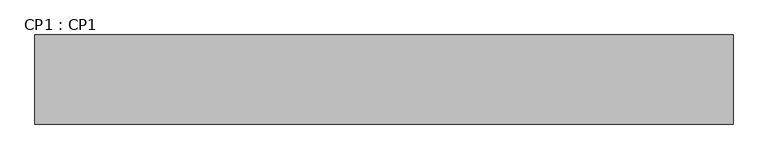
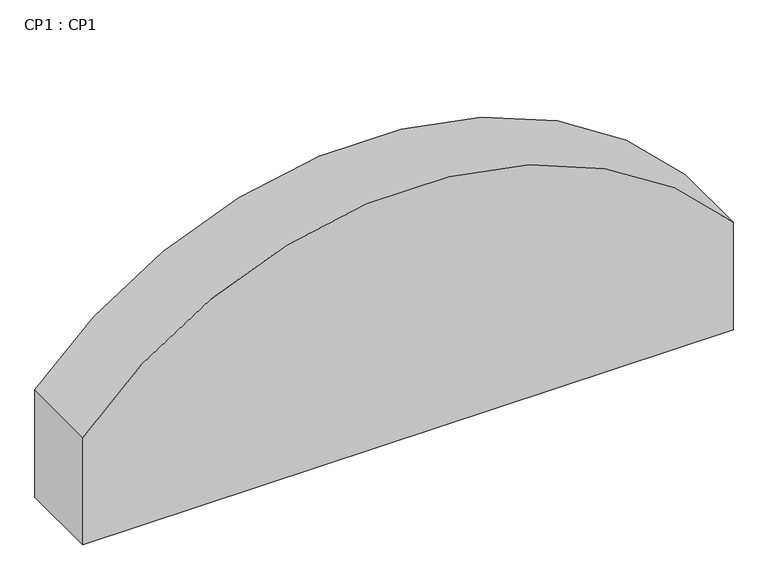
"""IFC4 building model written with IfcOpenShell, lengths in millimetres: beam geometry, CP1 : CP1."""

from ifc_helpers import new_model, si_unit, point, frame, frame_2d, origin, place, context, project, spatial, polyline, circle_curve, trimmed, segment, composite_curve, outline, extrude, source, transform, mapped, element, save


def cp1_cp1_2c4f1d20(model_context):
    return source(origin(), model_context, "Body", "SweptSolid", [
        extrude(outline(composite_curve([segment(trimmed(circle_curve(frame_2d((12608.2612414, 47833.2245512)), 3093.4758497), [point((14620.0, 50183.2245511))], [point((14620.0, 45483.2245512))], False, "CARTESIAN"), True, "CONTINUOUS"), segment(polyline([(14620.0, 45483.2245512), (13800.0, 45483.2245512), (13800.0, 50183.2245511), (14620.0, 50183.2245511)]), True, "CONTINUOUS")], self_intersect=False)), frame((0.0, -100.2551788, 0.0), z_axis=(0.0, 1.0, 0.0), x_axis=(0.0, 0.0, 1.0)), (0.0, 0.0, 1.0), 599.9551778),
    ])


if __name__ == "__main__":
    model = new_model("IFC4")
    model_context = context("Model", 3, world=origin())
    ifc_project = project(units=[si_unit("LENGTHUNIT", "METRE", prefix="MILLI")], contexts=[model_context])
    site = spatial("IfcSite", under=ifc_project)
    building = spatial("IfcBuilding", under=site)
    placement = place(None, origin())
    cp1_cp1_shape = cp1_cp1_2c4f1d20(model_context)
    element("IfcBeam", 1, ObjectType="CP1 : CP1", at=placement, inside=building, context=model_context, shape_type="MappedRepresentation", body=[
        mapped(cp1_cp1_shape, transform((0.0, 0.0, 0.0), x_axis=(1.0, 0.0, 0.0), y_axis=(0.0, 1.0, 0.0), z_axis=(0.0, 0.0, 1.0))),
    ])
    save(model, "model.ifc")
